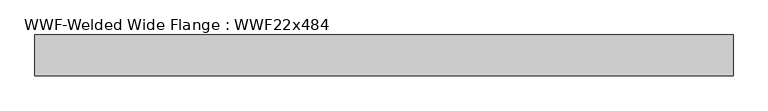
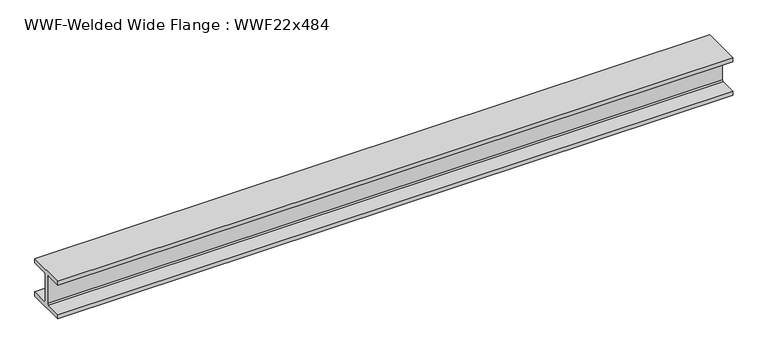
"""IFC4 building model written with IfcOpenShell, lengths in millimetres: member geometry, WWF-Welded Wide Flange : WWF22x484."""

from ifc_helpers import new_model, si_unit, frame, origin, place, context, project, spatial, polyline, outline, extrude, source, transform, mapped, element, save


def wwf_welded_wide_flange_wwf22x484_0dac382b(model_context):
    return source(origin(), model_context, "Body", "SweptSolid", [
        extrude(outline(polyline([(274.955, -214.9602), (274.955, -274.955), (-274.955, -274.955), (-274.955, -214.9602), (-47.625, -214.9602), (-29.9974, -197.3326), (-29.9974, 197.3326), (-47.625, 214.9602), (-274.955, 214.9602), (-274.955, 274.955), (274.955, 274.955), (274.955, 214.9602), (47.625, 214.9602), (29.9974, 197.3326), (29.9974, -197.3326), (47.625, -214.9602), (274.955, -214.9602)])), frame((-4712.345, 0.0, 0.0), z_axis=(1.0, 0.0, 0.0), x_axis=(0.0, 1.0, 0.0)), (0.0, 0.0, 1.0), 9374.652),
    ])


if __name__ == "__main__":
    model = new_model("IFC4")
    model_context = context("Model", 3, world=origin())
    ifc_project = project(units=[si_unit("LENGTHUNIT", "METRE", prefix="MILLI")], contexts=[model_context])
    site = spatial("IfcSite", under=ifc_project)
    building = spatial("IfcBuilding", under=site)
    placement = place(None, origin())
    wwf_welded_wide_flange_wwf22x484_shape = wwf_welded_wide_flange_wwf22x484_0dac382b(model_context)
    element("IfcMember", 1, ObjectType="WWF-Welded Wide Flange : WWF22x484", at=placement, inside=building, context=model_context, shape_type="MappedRepresentation", body=[
        mapped(wwf_welded_wide_flange_wwf22x484_shape, transform((0.0, 0.0, 0.0), x_axis=(1.0, 0.0, 0.0), y_axis=(0.0, 1.0, 0.0), z_axis=(0.0, 0.0, 1.0))),
    ])
    save(model, "model.ifc")

# Revit data of these elements
# Type "WWF-Welded Wide Flange : WWF22x484"
#   Assembly Code = "B10"
#   Nominal d = "12"
#   W = 484
#   Length [instance default] = 1524 mm
#   bf = 549.91 mm
#   d = 549.91 mm
#   k = 47.625 mm
#   tf = 59.995 mm
#   tw = 59.995 mm
#   A = 0.0922579 m²
#   Structural Material [instance default] = Steel ASTM A572
# Element 1 (IfcMember, "WWF-Welded Wide Flange : WWF22x484")
#   Materials on its faces: "Steel ASTM A572"
# Materials
#   "Steel ASTM A572": class "Metal", colour RGB 247 247 247, transparency 0, Description = "Structural steel, high strength low alloy, ASTM - A572 - 50", Cost = 0
